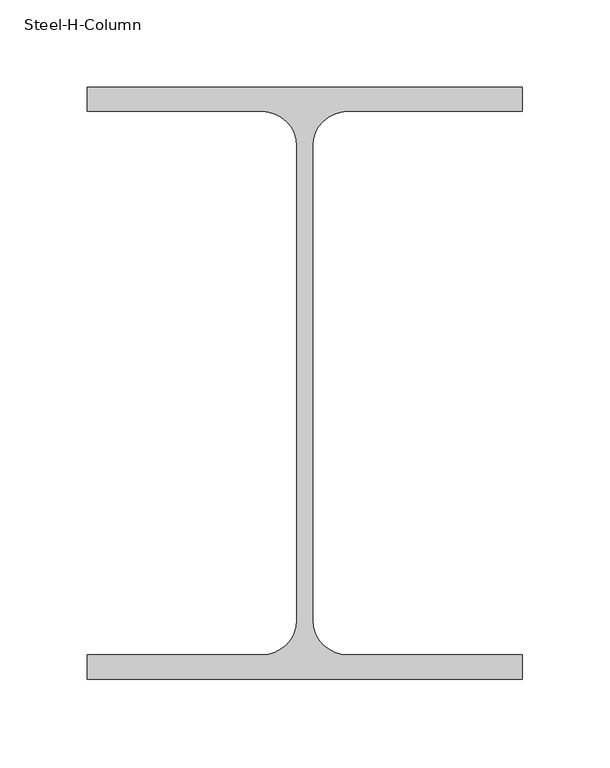
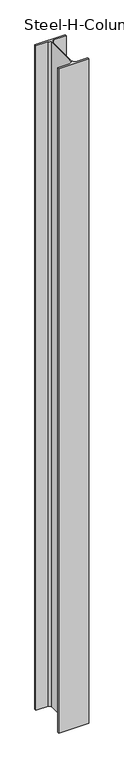
"""IFC4 building model written with IfcOpenShell, lengths in millimetres: column geometry, Steel-H-Column : CL121_H-340×250x9x14."""

import ifcopenshell
import ifcopenshell.guid

model = None  # the IFC model being written
_history = None  # IfcOwnerHistory: only IFC2X3 demands one
_inside = {}  # id of a spatial element -> (the spatial element, [elements in it])
_under = {}  # id of a project, library or spatial element -> (it, [spatial elements below it])
_declared = {}  # id of a project -> (the project, [libraries it declares])
_typed = {}  # id of a type object -> (the type object, [elements of that type])
_made_of = {}  # id of a material, layer set ... -> (it, [elements and type objects made of it])


def new_model(schema):
    """Start an empty IFC model of exactly this schema.

    Asked for "IFC4X3", IfcOpenShell would pick the latest addendum, in which some entities
    have other attributes; the version numbers below select the first issue.
    IFC2X3 requires an IfcOwnerHistory on every rooted entity: one is made here for all.
    """
    global model, _history
    if schema == "IFC4X3":
        model = ifcopenshell.file(schema_version=(4, 3, 0, 0))
    else:
        model = ifcopenshell.file(schema=schema)
    _inside.clear()
    _under.clear()
    _declared.clear()
    _typed.clear()
    _made_of.clear()
    _history = None
    if model.schema == "IFC2X3":
        org = make("IfcOrganization", Name="unknown")
        user = make(
            "IfcPersonAndOrganization",
            ThePerson=make("IfcPerson", FamilyName="unknown"),
            TheOrganization=org,
        )
        app = make(
            "IfcApplication",
            ApplicationDeveloper=org,
            Version="unknown",
            ApplicationFullName="unknown",
            ApplicationIdentifier="unknown",
        )
        _history = make(
            "IfcOwnerHistory",
            OwningUser=user,
            OwningApplication=app,
            ChangeAction="ADDED",
            CreationDate=0,
        )
    return model


def make(cls, **values):
    """One entity of the class cls with the attributes given. An attribute that is None is left unset."""
    return model.create_entity(
        cls, **{name: value for name, value in values.items() if value is not None}
    )


def rooted(cls, **values):
    """An entity with a GlobalId (a new one), such as an element, a storey or a relation."""
    return make(cls, GlobalId=ifcopenshell.guid.new(), OwnerHistory=_history, **values)


def si_unit(unit_type, name, prefix=None):
    """IfcSIUnit, for example si_unit("LENGTHUNIT", "METRE", prefix="MILLI")."""
    return make("IfcSIUnit", UnitType=unit_type, Prefix=prefix, Name=name)


def assignment(units):
    """IfcUnitAssignment: the units of a project."""
    return None if units is None else make("IfcUnitAssignment", Units=units)


def point(xyz):
    """IfcCartesianPoint."""
    return None if xyz is None else make("IfcCartesianPoint", Coordinates=xyz)


def direction(xyz):
    """IfcDirection."""
    return None if xyz is None else make("IfcDirection", DirectionRatios=xyz)


def frame(location, z_axis=None, x_axis=None):
    """IfcAxis2Placement3D, a coordinate frame: its origin and axes. An axis left out is left unset."""
    return make(
        "IfcAxis2Placement3D",
        Location=point(location),
        Axis=direction(z_axis),
        RefDirection=direction(x_axis),
    )


def frame_2d(location, x_axis=None):
    """IfcAxis2Placement2D, a coordinate frame in the plane: its origin and x axis."""
    return make(
        "IfcAxis2Placement2D", Location=point(location), RefDirection=direction(x_axis)
    )


def origin():
    """The frame at (0, 0, 0) with its axes left unset."""
    return frame((0.0, 0.0, 0.0))


def place(relative_to, where):
    """IfcLocalPlacement: puts the frame where relative to a parent placement (None: the world)."""
    return make(
        "IfcLocalPlacement", PlacementRelTo=relative_to, RelativePlacement=where
    )


def context(
    kind, dimensions, precision=None, world=None, true_north=None, identifier=None
):
    """IfcGeometricRepresentationContext, for example the 3D "Model" context."""
    return make(
        "IfcGeometricRepresentationContext",
        ContextIdentifier=identifier,
        ContextType=kind,
        CoordinateSpaceDimension=dimensions,
        Precision=precision,
        WorldCoordinateSystem=world,
        TrueNorth=true_north,
    )


def project(units=None, contexts=None):
    """IfcProject with its units and contexts."""
    return rooted(
        "IfcProject",
        Name="project",
        RepresentationContexts=contexts,
        UnitsInContext=assignment(units),
    )


def spatial(cls, under=None, at=None, **own):
    """A site, building, storey or space (cls), placed at a placement, below another one or the project."""
    s = rooted(cls, ObjectPlacement=at, **own)
    if under is not None:
        _under.setdefault(under.id(), (under, []))[1].append(s)
    return s


def polyline(points):
    """IfcPolyline through the points."""
    return make("IfcPolyline", Points=[point(p) for p in points])


def circle_curve(where, radius):
    """IfcCircle in the frame where."""
    return make("IfcCircle", Position=where, Radius=radius)


def trimmed(basis, trim1, trim2, sense, master):
    """IfcTrimmedCurve: the piece of a basis curve between two trims."""
    return make(
        "IfcTrimmedCurve",
        BasisCurve=basis,
        Trim1=trim1,
        Trim2=trim2,
        SenseAgreement=sense,
        MasterRepresentation=master,
    )


def segment(curve, same_sense, transition):
    """IfcCompositeCurveSegment."""
    return make(
        "IfcCompositeCurveSegment",
        Transition=transition,
        SameSense=same_sense,
        ParentCurve=curve,
    )


def composite_curve(segments, self_intersect=None):
    """IfcCompositeCurve: segments joined end to end."""
    return make("IfcCompositeCurve", Segments=segments, SelfIntersect=self_intersect)


def outline(outer, holes=None, kind="AREA"):
    """IfcArbitraryClosedProfileDef: a profile drawn as a closed curve; with holes, ...WithVoids."""
    if holes is None:
        return make("IfcArbitraryClosedProfileDef", ProfileType=kind, OuterCurve=outer)
    return make(
        "IfcArbitraryProfileDefWithVoids",
        ProfileType=kind,
        OuterCurve=outer,
        InnerCurves=holes,
    )


def extrude(swept, where, along, depth):
    """IfcExtrudedAreaSolid: the profile swept, set in the frame where, extruded along a direction by depth."""
    return make(
        "IfcExtrudedAreaSolid",
        SweptArea=swept,
        Position=where,
        ExtrudedDirection=direction(along),
        Depth=depth,
    )


def shape(context_of_items, identifier, shape_type, items):
    """IfcShapeRepresentation: the items that make up one representation, for example the "Body"."""
    return make(
        "IfcShapeRepresentation",
        ContextOfItems=context_of_items,
        RepresentationIdentifier=identifier,
        RepresentationType=shape_type,
        Items=items,
    )


def source(mapping_origin, context_of_items, identifier, shape_type, items):
    """IfcRepresentationMap: a shape defined once, which mapped items show again and again."""
    return make(
        "IfcRepresentationMap",
        MappingOrigin=mapping_origin,
        MappedRepresentation=shape(context_of_items, identifier, shape_type, items),
    )


def transform(
    local_origin,
    x_axis=None,
    y_axis=None,
    z_axis=None,
    scale=None,
    scale2=None,
    scale3=None,
    uniform=True,
):
    """IfcCartesianTransformationOperator3D, or its non-uniform kind. x_axis, y_axis, z_axis: its Axis1, 2, 3."""
    if uniform:
        return make(
            "IfcCartesianTransformationOperator3D",
            Axis1=direction(x_axis),
            Axis2=direction(y_axis),
            LocalOrigin=point(local_origin),
            Scale=scale,
            Axis3=direction(z_axis),
        )
    return make(
        "IfcCartesianTransformationOperator3DnonUniform",
        Axis1=direction(x_axis),
        Axis2=direction(y_axis),
        LocalOrigin=point(local_origin),
        Scale=scale,
        Axis3=direction(z_axis),
        Scale2=scale2,
        Scale3=scale3,
    )


def mapped(mapping_source, mapping_target):
    """IfcMappedItem: shows the shape of a source again, moved by a transform."""
    return make(
        "IfcMappedItem", MappingSource=mapping_source, MappingTarget=mapping_target
    )


def made_of(thing, what):
    """Note that an element or type object is made of a material, layer set ...; save() writes the relation."""
    if what is not None:
        _made_of.setdefault(what.id(), (what, []))[1].append(thing)
    return thing


def element(
    cls,
    number,
    at=None,
    inside=None,
    cuts=None,
    type_object=None,
    material=None,
    context=None,
    identifier="Body",
    shape_type=None,
    held_by="IfcProductDefinitionShape",
    body=None,
    shapes=None,
    **own,
):
    """One element of the class cls, such as IfcWall. Its Tag is "e" and its number.

    at: its placement. inside: the storey or other place that contains it. cuts: it is an
    opening in that element (IfcRelVoidsElement). A single representation is given by context,
    identifier, shape_type and body (its items); several are given by shapes. held_by: the class
    of the entity that holds the representations. save() writes the other relations.
    """
    e = rooted(cls, Tag="e%d" % number, ObjectPlacement=at, **own)
    if body is not None:
        shapes = [shape(context, identifier, shape_type, body)]
    if shapes is not None:
        e.Representation = make(held_by, Representations=shapes)
    if inside is not None:
        _inside.setdefault(inside.id(), (inside, []))[1].append(e)
    if cuts is not None:
        rooted(
            "IfcRelVoidsElement", RelatingBuildingElement=cuts, RelatedOpeningElement=e
        )
    if type_object is not None:
        _typed.setdefault(type_object.id(), (type_object, []))[1].append(e)
    return made_of(e, material)


def aggregate(whole, parts):
    """IfcRelAggregates: a whole, such as a stair, and the parts it consists of."""
    return rooted("IfcRelAggregates", RelatingObject=whole, RelatedObjects=parts)


def save(model, path):
    """Write the relations noted so far, then the file.

    IfcRelAggregates (storeys below a building ...), IfcRelContainedInSpatialStructure (elements
    in a storey), IfcRelDefinesByType, IfcRelAssociatesMaterial and IfcRelDeclares: one each for
    every whole, place, type object, material and project.
    """
    for whole, parts in _under.values():
        aggregate(whole, parts)
    for where, things in _inside.values():
        rooted(
            "IfcRelContainedInSpatialStructure",
            RelatedElements=things,
            RelatingStructure=where,
        )
    for kind, things in _typed.values():
        rooted("IfcRelDefinesByType", RelatedObjects=things, RelatingType=kind)
    for what, things in _made_of.values():
        rooted("IfcRelAssociatesMaterial", RelatedObjects=things, RelatingMaterial=what)
    for by, libraries in _declared.values():
        rooted("IfcRelDeclares", RelatingContext=by, RelatedDefinitions=libraries)
    model.write(path)


def steel_h_column_09ca9198(model_context):
    return source(origin(), model_context, "Body", "SweptSolid", [
        extrude(outline(composite_curve([segment(polyline([(125.0, 170.0), (125.0, 156.0), (24.5, 156.0)]), True, "CONTINUOUS"), segment(trimmed(circle_curve(frame_2d((24.5, 136.0)), 20.0), [point((24.5, 156.0))], [point((4.5, 136.0))], True, "CARTESIAN"), True, "CONTINUOUS"), segment(polyline([(4.5, 136.0), (4.5, -136.0)]), True, "CONTINUOUS"), segment(trimmed(circle_curve(frame_2d((24.5, -136.0)), 20.0), [point((4.5, -136.0))], [point((24.5, -156.0))], True, "CARTESIAN"), True, "CONTINUOUS"), segment(polyline([(24.5, -156.0), (125.0, -156.0), (125.0, -170.0), (-125.0, -170.0), (-125.0, -156.0), (-24.5, -156.0)]), True, "CONTINUOUS"), segment(trimmed(circle_curve(frame_2d((-24.5, -136.0)), 20.0), [point((-24.5, -156.0))], [point((-4.5, -136.0))], True, "CARTESIAN"), True, "CONTINUOUS"), segment(polyline([(-4.5, -136.0), (-4.5, 136.0)]), True, "CONTINUOUS"), segment(trimmed(circle_curve(frame_2d((-24.5, 136.0)), 20.0), [point((-4.5, 136.0))], [point((-24.5, 156.0))], True, "CARTESIAN"), True, "CONTINUOUS"), segment(polyline([(-24.5, 156.0), (-125.0, 156.0), (-125.0, 170.0), (125.0, 170.0)]), True, "CONTINUOUS")], self_intersect=False)), frame((0.0, 0.0, 200.0), z_axis=(0.0, 0.0, 1.0), x_axis=(1.0, 0.0, 0.0)), (0.0, 0.0, 1.0), 5800.0),
    ])


if __name__ == "__main__":
    model = new_model("IFC4")
    model_context = context("Model", 3, world=origin())
    ifc_project = project(units=[si_unit("LENGTHUNIT", "METRE", prefix="MILLI")], contexts=[model_context])
    site = spatial("IfcSite", under=ifc_project)
    building = spatial("IfcBuilding", under=site)
    placement = place(None, origin())
    steel_h_column_shape = steel_h_column_09ca9198(model_context)
    element("IfcColumn", 1, ObjectType="Steel-H-Column : CL121_H-340×250x9x14", at=placement, inside=building, context=model_context, shape_type="MappedRepresentation", body=[
        mapped(steel_h_column_shape, transform((0.0, 0.0, 0.0), x_axis=(1.0, 0.0, 0.0), y_axis=(0.0, 1.0, 0.0), z_axis=(0.0, 0.0, 1.0))),
    ])
    save(model, "model.ifc")

# Revit data of these elements
# Project information
#   Project ISM Data = "<?xml version=\"1.0\" encoding=\"utf-16\"?><ism schema_version=\"03.00\"><section_positioning><element family_name=\"CO_RC_REC\" symbol_name=\"CCC12_Rec_450x450\" section_id=\"F2ADF140-E21A-4820-8170-6F63D956DCAD\" category=\"OST_StructuralColumns\" mirror_y=\"0\" mirror_x=\"0\" /><element family_name=\"CO_RC_REC\" symbol_name=\"CCC12_Rec_450x450\" section_id=\"B35A310E-4F33-462b-819C-3ADD300C0CEB\" category=\"OST_StructuralColumns\" mirror_y=\"0\" mirror_x=\"0\" /><element family_name=\"CO_RC_REC\" symbol_name=\"CCC12_Rec_450x450\" section_id=\"711054EC-0DB2-46e3-AD20-004560300C00\" category=\"OST_StructuralColumns\" mirror_y=\"0\" mirror_x=\"0\" /><element family_name=\"CO_RC_REC\" symbol_name=\"300 x 450\" section_id=\"B5C54EC9-8EBD-4860-AB72-EF5791AED394\" category=\"OST_StructuralColumns\" mirror_y=\"0\" mirror_x=\"0\" /><element family_name=\"GI_RC_C\" symbol_name=\"SGC11_400x500\" section_id=\"0A7B8D02-9EA4-4aa9-A41A-E30BB5B6B6C5\" category=\"OST_StructuralFraming\" mirror_y=\"0\" mirror_x=\"0\" /><element family_name=\"GI_RC_C\" symbol_name=\"SGC11_400x500\" section_id=\"714BBD27-DB58-47da-B54C-5806291C2D3C\" category=\"OST_StructuralFraming\" mirror_y=\"0\" mirror_x=\"0\" /><element family_name=\"GI_RC_C\" symbol_name=\"SGC11_400x500\" section_id=\"F36E62C1-13EE-4807-A3C1-899E23E0BEDE\" category=\"OST_StructuralFraming\" mirror_y=\"0\" mirror_x=\"0\" /><element family_name=\"GI_RC_C\" symbol_name=\"SGC11_400x500\" section_id=\"F5448801-679E-44d6-8F46-E676344F8165\" category=\"OST_StructuralFraming\" mirror_y=\"0\" mirror_x=\"0\" /><element family_name=\"GI_RC_C\" symbol_name=\"SGC11_400x600\" section_id=\"05D74241-6318-4cac-95F5-7B878260D5B5\" category=\"OST_StructuralFraming\" mirror_y=\"0\" mirror_x=\"0\" /><element family_name=\"GI_RC_C\" symbol_name=\"SGC11_400x500\" section_id=\"846DCB0C-E06B-4978-9D43-E1CC0FDE7595\" category=\"OST_StructuralFraming\" mirror_y=\"0\" mirror_x=\"0\" /><element family_name=\"GI_RC_C\" symbol_name=\"SGC11_400x500\" section_id=\"2ADF82B8-986D-4f44-85DE-89D921292160\" category=\"OST_StructuralFraming\" mirror_y=\"0\" mirror_x=\"0\" /><element family_name=\"GI_RC_C\" symbol_name=\"SGC11_400x500\" section_id=\"7AF371ED-051B-4a30-8826-11F11C212B73\" category=\"OST_StructuralFraming\" mirror_y=\"0\" mirror_x=\"0\" /><element family_name=\"GI_RC_C\" symbol_name=\"SGC11_400x500\" section_id=\"2FE74006-ADDA-412f-A522-853919E62B4D\" category=\"OST_StructuralFraming\" mirror_y=\"0\" mirror_x=\"0\" /><element family_name=\"GI_RC_C\" symbol_name=\"SGC11_400x500\" section_id=\"09B63641-D581-4a6c-A18E-54C17EC989A4\" category=\"OST_StructuralFraming\" mirror_y=\"0\" mirror_x=\"0\" /><element family_name=\"GI_RC_C\" symbol_name=\"SGC11_400x500\" section_id=\"0DD6B52A-77D0-45a1-82B1-8236ED57078C\" category=\"OST_StructuralFraming\" mirror_y=\"0\" mirror_x=\"0\" /><element family_name=\"GI_RC_C\" symbol_name=\"SGC11_400x500\" section_id=\"35D311D2-DEB8-4469-97DE-110B6DF5B84D\" category=\"OST_StructuralFraming\" mirror_y=\"0\" mirror_x=\"0\" /><element family_name=\"GI_RC_C\" symbol_name=\"SGC11_400x500\" section_id=\"0D3CCDE5-CFF9-431b-A4BD-01BF6636D6BD\" category=\"OST_StructuralFraming\" mirror_y=\"0\" mirror_x=\"0\" /><element family_name=\"GI_RC_C\" symbol_name=\"SGC11_400x500\" section_id=\"C62B2A5B-024A-47ac-B030-C17A67E64A7B\" category=\"OST_StructuralFraming\" mirror_y=\"0\" mirror_x=\"0\" /><element family_name=\"GI_RC_C\" symbol_name=\"SGC11_400x500\" section_id=\"944C6E43-E607-48c3-8358-9E6CB88346E7\" category=\"OST_StructuralFraming\" mirror_y=\"0\" mirror_x=\"0\" /><element family_name=\"GI_RC_C\" symbol_name=\"SGC11_400x500\" section_id=\"A4B1F42D-B1C2-4ad2-8AD6-DB0D5E05998D\" category=\"OST_StructuralFraming\" mirror_y=\"0\" mirror_x=\"0\" /><element family_name=\"GI_RC_C\" symbol_name=\"SGC11_400x500\" section_id=\"007E6C70-1139-4b48-B003-C76FAD4C249A\" category=\"OST_StructuralFraming\" mirror_y=\"0\" mirror_x=\"0\" /><element family_name=\"GI_RC_C\" symbol_name=\"SGC11_400x500\" section_id=\"9941AC94-F03A-464c-9912-04590E0C31E0\" category=\"OST_StructuralFraming\" mirror_y=\"0\" mirror_x=\"0\" /><element family_name=\"GI_RC_C\" symbol_name=\"SGC11_400x500\" section_id=\"CFD98B8D-8FF4-4e71-A909-0FE7DBCE924E\" category=\"OST_StructuralFraming\" mirror_y=\"0\" mirror_x=\"0\" /><element family_name=\"GI_RC_C\" symbol_name=\"SGC11_400x500\" section_id=\"58262161-98E6-45c8-B2BD-4508105FF662\" category=\"OST_StructuralFraming\" mirror_y=\"0\" mirror_x=\"0\" /><element family_name=\"GI_RC_C\" symbol_name=\"SGC11_400x500\" section_id=\"66AB4841-610A-4883-97F7-1282A56484E1\" category=\"OST_StructuralFraming\" mirror_y=\"0\" mirror_x=\"0\" /><element family_name=\"GI_RC_C\" symbol_name=\"SGC11_400x500\" section_id=\"D2B324BE-BBD6-49da-9730-60EA7AD4D3A0\" category=\"OST_StructuralFraming\" mirror_y=\"0\" mirror_x=\"0\" /><element family_name=\"GI_RC_C\" symbol_name=\"SGC11_400x500\" section_id=\"92A8ECE7-C053-46b1-92ED-F2C041617E7B\" category=\"OST_StructuralFraming\" mirror_y=\"0\" mirror_x=\"0\" /><element family_name=\"GI_RC_C\" symbol_name=\"SGC11_400x500\" section_id=\"B4C4BDB0-65C4-4016-9C78-DBD77E229523\" category=\"OST_StructuralFraming\" mirror_y=\"0\" mirror_x=\"0\" /><element family_name=\"GI_RC_C\" symbol_name=\"SGC11_400x500\" section_id=\"57270646-162F-4c83-BDB7-A5FBEA9120BD\" category=\"OST_StructuralFraming\" mirror_y=\"0\" mirror_x=\"0\" /><element family_name=\"GI_RC_C\" symbol_name=\"SGC11_400x500\" section_id=\"BDEF733F-00AA-4eee-B6C6-50229FC1D236\" category=\"OST_StructuralFraming\" mirror_y=\"0\" mirror_x=\"0\" /><element family_name=\"GI_RC_C\" symbol_name=\"SGC11_400x500\" section_id=\"84A94E1E-3074-40f4-9690-97191755F019\" category=\"OST_StructuralFraming\" mirror_y=\"0\" mirror_x=\"0\" /><element family_name=\"GI_RC_C\" symbol_name=\"SGC11_400x500\" section_id=\"8A7D913D-7967-4718-912D-B83DF0AD2EDD\" category=\"OST_StructuralFraming\" mirror_y=\"0\" mirror_x=\"0\" /><element family_name=\"GI_RC_C\" symbol_name=\"SGC11_400x500\" section_id=\"83553D70-90FA-469c-B5C3-EF03F3FC6475\" category=\"OST_StructuralFraming\" mirror_y=\"0\" mirror_x=\"0\" /><element family_name=\"GI_RC_C\" symbol_name=\"SGC11_400x500\" section_id=\"6880C1E4-C50B-4c1b-B61C-23F2D8C46873\" category=\"OST_StructuralFraming\" mirror_y=\"0\" mirror_x=\"0\" /><element family_name=\"GI_RC_C\" symbol_name=\"SGC11_400x500\" section_id=\"08594C43-CD40-47de-A3BA-8BFB47F64994\" category=\"OST_StructuralFraming\" mirror_y=\"0\" mirror_x=\"0\" /><element family_name=\"GI_RC_C\" symbol_name=\"SGC11_400x500\" section_id=\"7D2E11FA-A5E1-4434-B9BE-AABA1A16CA03\" category=\"OST_StructuralFraming\" mirror_y=\"0\" mirror_x=\"0\" /><element family_name=\"GI_RC_C\" symbol_name=\"SGC11_400x500\" section_id=\"D892DFA4-5441-4ad2-A390-253492293B1B\" category=\"OST_StructuralFraming\" mirror_y=\"0\" mirror_x=\"0\" /><element family_name=\"GI_RC_C\" symbol_name=\"SGC11_400x500\" section_id=\"E5A32FE6-89C4-49f1-B3B9-1CABE7C48A4D\" category=\"OST_StructuralFraming\" mirror_y=\"0\" mirror_x=\"0\" /><element family_name=\"GI_RC_C\" symbol_name=\"SGC11_400x500\" section_id=\"8AE872C2-5DBE-47c5-934B-7E964A84B589\" category=\"OST_StructuralFraming\" mirror_y=\"0\" mirror_x=\"0\" /><element family_name=\"GI_RC_C\" symbol_name=\"SGC11_400x500\" section_id=\"3C847B60-488A-4604-A400-16A3A65E919B\" category=\"OST_StructuralFraming\" mirror_y=\"0\" mirror_x=\"0\" /><element family_name=\"GI_RC_C\" symbol_name=\"SGC11_400x500\" section_id=\"DBEC432A-3F7B-4266-AD99-2A937DC70BCF\" category=\"OST_StructuralFraming\" mirror_y=\"0\" mirror_x=\"0\" /><element family_name=\"GI_RC_C\" symbol_name=\"SGC11_400x500\" section_id=\"59403DD6-7A51-48aa-A3BE-962457E6F10E\" category=\"OST_StructuralFraming\" mirror_y=\"0\" mirror_x=\"0\" /><element family_name=\"GI_RC_C\" symbol_name=\"SGC11_400x500\" section_id=\"11CDDF5D-38B6-43b2-A291-FC188BE232BC\" category=\"OST_StructuralFraming\" mirror_y=\"0\" mirror_x=\"0\" /><element family_name=\"GI_RC_C\" symbol_name=\"SGC11_400x500\" section_id=\"10BF2843-EFC9-4136-933C-5B270D970277\" category=\"OST_StructuralFraming\" mirror_y=\"0\" mirror_x=\"0\" /><element family_name=\"GI_RC_C\" symbol_name=\"SGC11_400x500\" section_id=\"E1B09A9C-F6C6-47d9-976B-E313C0E3F52B\" category=\"OST_StructuralFraming\" mirror_y=\"0\" mirror_x=\"0\" /><element family_name=\"GI_RC_C\" symbol_name=\"SGC11_400x500\" section_id=\"A3A22EC3-26C8-4588-A0AB-AFAE02DF267E\" category=\"OST_StructuralFraming\" mirror_y=\"0\" mirror_x=\"0\" /><element family_name=\"GI_RC_C\" symbol_name=\"SGC11_400x500\" section_id=\"114828FC-BDC1-4343-9119-BCB5395DAA64\" category=\"OST_StructuralFraming\" mirror_y=\"0\" mirror_x=\"0\" /><element family_name=\"GI_RC_C\" symbol_name=\"SGC11_400x500\" section_id=\"797626F9-3558-4623-826F-15FB93088CB3\" category=\"OST_StructuralFraming\" mirror_y=\"0\" mirror_x=\"0\" /><element family_name=\"GI_RC_C\" symbol_name=\"SGC11_400x500\" section_id=\"4BF369CD-DF09-4346-96CB-C6C6380A2599\" category=\"OST_StructuralFraming\" mirror_y=\"0\" mirror_x=\"0\" /><element family_name=\"GI_RC_C\" symbol_name=\"SGC11_400x500\" section_id=\"722B46BA-61C4-44a1-9ECF-325B60B6688D\" category=\"OST_StructuralFraming\" mirror_y=\"0\" mirror_x=\"0\" /><element family_name=\"GI_RC_C\" symbol_name=\"SGC11_400x500\" section_id=\"C33DBE84-19C1-4379-AB6E-A41F7420F18C\" category=\"OST_StructuralFraming\" mirror_y=\"0\" mirror_x=\"0\" /><element family_name=\"GI_RC_C\" symbol_name=\"SGC11_400x500\" section_id=\"1F2D3B75-66F2-4d88-A1DD-647969477B86\" category=\"OST_StructuralFraming\" mirror_y=\"0\" mirror_x=\"0\" /><element family_name=\"GI_RC_C\" symbol_name=\"SGC11_400x500\" section_id=\"DFBF96B2-410A-4f39-80C4-D8CF78561C93\" category=\"OST_StructuralFraming\" mirror_y=\"0\" mirror_x=\"0\" /><element family_name=\"GI_RC_C\" symbol_name=\"SGC11_400x500\" section_id=\"D6793CD3-AB64-417c-9C28-8B18A0A2D336\" category=\"OST_StructuralFraming\" mirror_y=\"0\" mirror_x=\"0\" /><element family_name=\"GI_RC_C\" symbol_name=\"SGC11_400x500\" section_id=\"90884AC0-EA00-4caa-86E1-E6B886FD90ED\" category=\"OST_StructuralFraming\" mirror_y=\"0\" mirror_x=\"0\" /><element family_name=\"GI_RC_C\" symbol_name=\"SGC11_400x500\" section_id=\"64BC7B89-F7C8-4dae-A5C8-F10DF9E5F6BA\" category=\"OST_StructuralFraming\" mirror_y=\"0\" mirror_x=\"0\" /><element family_name=\"GI_RC_C\" symbol_name=\"SGC11_400x500\" section_id=\"D82E4D85-2728-40e5-9F60-1C7FB2990D78\" category=\"OST_StructuralFraming\" mirror_y=\"0\" mirror_x=\"0\" /><element family_name=\"GI_RC_C\" symbol_name=\"SGC11_400x500\" section_id=\"1E6D05B9-BF84-4669-AA27-948ADA1D511E\" category=\"OST_StructuralFraming\" mirror_y=\"0\" mirror_x=\"0\" /><element family_name=\"GI_RC_C\" symbol_name=\"SGC11_400x500\" section_id=\"73608CB2-EB94-466e-883D-814030EF49D6\" category=\"OST_StructuralFraming\" mirror_y=\"0\" mirror_x=\"0\" /><element family_name=\"GI_RC_C\" symbol_name=\"SGC11_400x500\" section_id=\"4EAF07EF-4E08-4065-9F08-BF69D4413867\" category=\"OST_StructuralFraming\" mirror_y=\"1\" mirror_x=\"1\" /></section_positioning><surface_member_mappings /><element_binding><element revit_id=\"0aa8b22b-49cd-4eb2-b994-d423f7aad482-0014435e\" ism_id=\"637A3C89-B4B9-4EE4-9E04-FF73E7A5771D\" /><element revit_id=\"af7cfdda-f71a-4a09-bb03-63e0c16d5d93-00152efa\" ism_id=\"088C1743-AFAE-4D55-B14F-2330F3A79060\" /><element revit_id=\"af7cfdda-f71a-4a09-bb03-63e0c16d5d93-00152efc\" ism_id=\"38278b30-864a-4bde-bfee-6c2d4309b281\" /><element revit_id=\"af7cfdda-f71a-4a09-bb03-63e0c16d5d93-00152eff\" ism_id=\"e2895b00-887b-4cf1-92a9-c4855f67b579\" /><element revit_id=\"af7cfdda-f71a-4a09-bb03-63e0c16d5d93-00152f02\" ism_id=\"a6b13b86-1938-47ee-8937-754844bb71d9\" /><element revit_id=\"af7cfdda-f71a-4a09-bb03-63e0c16d5d93-00152f05\" ism_id=\"b3cdb4ae-01be-49a8-8521-dfb37fcb7a09\" /><element revit_id=\"af7cfdda-f71a-4a09-bb03-63e0c16d5d93-00152f08\" ism_id=\"0a200294-2d0f-43b2-a10b-c345be42008c\" /><element revit_id=\"af7cfdda-f71a-4a09-bb03-63e0c16d5d
#     93-00152f0a\" ism_id=\"434ac00d-0b75-408a-b526-bf8655b26baf\" /><element revit_id=\"af7cfdda-f71a-4a09-bb03-63e0c16d5d93-00152f0c\" ism_id=\"5e4f7e2a-2154-47cc-93bc-24e7bd197632\" /><element revit_id=\"af7cfdda-f71a-4a09-bb03-63e0c16d5d93-00152f0e\" ism_id=\"f1998cd9-044c-4f7a-99e6-248bc5b45dba\" /><element revit_id=\"af7cfdda-f71a-4a09-bb03-63e0c16d5d93-00152f10\" ism_id=\"6ca0e144-6dd7-4824-b6a4-c3599ffcc64c\" /><element revit_id=\"af7cfdda-f71a-4a09-bb03-63e0c16d5d93-00152f12\" ism_id=\"173f1f07-ca52-4750-b7f6-1ef0180c36ba\" /><element revit_id=\"af7cfdda-f71a-4a09-bb03-63e0c16d5d93-00152f15\" ism_id=\"29a619d1-86ac-46c7-a220-2e78769b313e\" /><element revit_id=\"af7cfdda-f71a-4a09-bb03-63e0c16d5d93-00152f17\" ism_id=\"de21b25d-6b5e-4da6-89ee-8b671f1287ec\" /><element revit_id=\"af7cfdda-f71a-4a09-bb03-63e0c16d5d93-00152f19\" ism_id=\"70cdf538-eeaa-48c4-9315-181e56578638\" /><element revit_id=\"af7cfdda-f71a-4a09-bb03-63e0c16d5d93-00152f1b\" ism_id=\"49734cf8-a963-4163-b104-a25bff74fff0\" /><element revit_id=\"af7cfdda-f71a-4a09-bb03-63e0c16d5d93-00152f1d\" ism_id=\"a5a98e28-e98d-4759-bcab-d40632bfc19f\" /><element revit_id=\"af7cfdda-f71a-4a09-bb03-63e0c16d5d93-00152f1f\" ism_id=\"ab6af08f-90da-4d2f-a66a-db65621b8e94\" /><element revit_id=\"af7cfdda-f71a-4a09-bb03-63e0c16d5d93-00152f21\" ism_id=\"a65b64ab-134d-4223-82b7-5e66d90bc276\" /><element revit_id=\"af7cfdda-f71a-4a09-bb03-63e0c16d5d93-00152f23\" ism_id=\"6a1f317f-8940-4af8-9522-8e6c47c0c3a6\" /><element revit_id=\"af7cfdda-f71a-4a09-bb03-63e0c16d5d93-00152f25\" ism_id=\"880c6aab-7058-4382-9d83-6c759bdcf822\" /><element revit_id=\"af7cfdda-f71a-4a09-bb03-63e0c16d5d93-00152f27\" ism_id=\"555977b1-6494-4ee8-b235-8bae97762787\" /><element revit_id=\"af7cfdda-f71a-4a09-bb03-63e0c16d5d93-00152f29\" ism_id=\"66c9b467-8c65-4f1e-9542-95b43d793e9b\" /><element revit_id=\"af7cfdda-f71a-4a09-bb03-63e0c16d5d93-00152f2b\" ism_id=\"217a9ce2-64ab-4115-836e-06014fa1b21e\" /><element revit_id=\"af7cfdda-f71a-4a09-bb03-63e0c16d5d93-00152f2d\" ism_id=\"f7fc30da-832d-44e7-bab3-dd115d25639e\" /><element revit_id=\"af7cfdda-f71a-4a09-bb03-63e0c16d5d93-00152f2f\" ism_id=\"715eb46c-1b8d-4226-a7c6-6c6c165bf34d\" /><element revit_id=\"af7cfdda-f71a-4a09-bb03-63e0c16d5d93-00152f31\" ism_id=\"ef53c2b2-6fcf-42d2-96ea-f30a899bf64f\" /><element revit_id=\"af7cfdda-f71a-4a09-bb03-63e0c16d5d93-00152f34\" ism_id=\"1aefa093-18ee-4a97-8178-1b1fb4b7aceb\" /><element revit_id=\"af7cfdda-f71a-4a09-bb03-63e0c16d5d93-00152f38\" ism_id=\"262f02a9-64ca-487b-befd-4b58d44dffa7\" /><element revit_id=\"af7cfdda-f71a-4a09-bb03-63e0c16d5d93-00152f3b\" ism_id=\"6f2442a8-c4c0-4b53-9d7f-7059d6ededd2\" /><element revit_id=\"af7cfdda-f71a-4a09-bb03-63e0c16d5d93-00152f3e\" ism_id=\"dd838df4-69c7-406c-93e1-418c01f5734f\" /><element revit_id=\"af7cfdda-f71a-4a09-bb03-63e0c16d5d93-00152f40\" ism_id=\"9dec5077-28a7-4c32-95d2-08813de6a916\" /><element revit_id=\"af7cfdda-f71a-4a09-bb03-63e0c16d5d93-00152f42\" ism_id=\"9370ae5f-9277-4bb3-917b-cb3f318800a8\" /><element revit_id=\"af7cfdda-f71a-4a09-bb03-63e0c16d5d93-00152f44\" ism_id=\"0f3f2c81-58b4-4698-b1be-75061a4a2ae1\" /><element revit_id=\"af7cfdda-f71a-4a09-bb03-63e0c16d5d93-00152f46\" ism_id=\"95dca10f-6510-4ae7-a23e-7a1fd6939662\" /><element revit_id=\"af7cfdda-f71a-4a09-bb03-63e0c16d5d93-00152f49\" ism_id=\"83bad907-6a1c-4702-9990-a1a9c13d0160\" /><element revit_id=\"af7cfdda-f71a-4a09-bb03-63e0c16d5d93-00152f4d\" ism_id=\"7dba72dc-0de8-457c-8d3c-9c80941133ff\" /><element revit_id=\"af7cfdda-f71a-4a09-bb03-63e0c16d5d93-00152f51\" ism_id=\"a6cf3de2-949b-45b4-8029-061e06e5ab91\" /><element revit_id=\"af7cfdda-f71a-4a09-bb03-63e0c16d5d93-00152f54\" ism_id=\"77af5754-dd62-4c90-accb-d0b9405b5baf\" /><element revit_id=\"af7cfdda-f71a-4a09-bb03-63e0c16d5d93-00152f56\" ism_id=\"6461cb37-823d-49bb-bea2-3dbd4db85a81\" /><element revit_id=\"af7cfdda-f71a-4a09-bb03-63e0c16d5d93-00152f59\" ism_id=\"e2f2909f-27bc-426e-b2db-27b1217d3560\" /><element revit_id=\"af7cfdda-f71a-4a09-bb03-63e0c16d5d93-00152f5b\" ism_id=\"46c410de-fc65-4593-ae24-da1a154b45fb\" /><element revit_id=\"af7cfdda-f71a-4a09-bb03-63e0c16d5d93-00152f5d\" ism_id=\"d7d73cf7-a31f-421c-bc39-3ba338a334b1\" /><element revit_id=\"af7cfdda-f71a-4a09-bb03-63e0c16d5d93-00152f61\" ism_id=\"6bd81f7b-5fd8-4f19-ad3a-4e009274854c\" /><element revit_id=\"af7cfdda-f71a-4a09-bb03-63e0c16d5d93-00152f64\" ism_id=\"f25b9af0-504f-4aaf-a359-d2bc9d32b683\" /><element revit_id=\"af7cfdda-f71a-4a09-bb03-63e0c16d5d93-00152f66\" ism_id=\"f143dcd3-1cc7-47ae-b4ed-c960a7d1349c\" /><element revit_id=\"af7cfdda-f71a-4a09-bb03-63e0c16d5d93-00152f68\" ism_id=\"296e8d7f-a89b-405a-b793-fc1ea4b11be5\" /><element revit_id=\"af7cfdda-f71a-4a09-bb03-63e0c16d5d93-00152f6b\" ism_id=\"48b24488-3184-439c-b285-73e81edfef17\" /><element revit_id=\"af7cfdda-f71a-4a09-bb03-63e0c16d5d93-00152f6e\" ism_id=\"0db0ccd4-631c-4972-aad8-2fd483c55629\" /><element revit_id=\"af7cfdda-f71a-4a09-bb03-63e0c16d5d93-00152f71\" ism_id=\"ee51bd40-01d8-4a48-92c6-90509a96cad2\" /><element revit_id=\"af7cfdda-f71a-4a09-bb03-63e0c16d5d93-00152f73\" ism_id=\"e5c66ce6-ca9d-4591-9d75-5348307a88bc\" /><element revit_id=\"af7cfdda-f71a-4a09-bb03-63e0c16d5d93-00152f75\" ism_id=\"892d82ae-6f73-4af5-8575-78955f2b6c3b\" /><element revit_id=\"af7cfdda-f71a-4a09-bb03-63e0c16d5d93-00152f78\" ism_id=\"cb5b2a2e-5551-4b87-9d0b-6382c09e6ce2\" /><element revit_id=\"af7cfdda-f71a-4a09-bb03-63e0c16d5d93-00152f7c\" ism_id=\"1177c4ab-d04b-426b-80ba-afa1f1403e20\" /><element revit_id=\"af7cfdda-f71a-4a09-bb03-63e0c16d5d93-00152f7f\" ism_id=\"235d8a18-f10a-44ad-8945-ebb2f02646fa\" /><element revit_id=\"af7cfdda-f71a-4a09-bb03-63e0c16d5d93-00152f83\" ism_id=\"6127db9d-7d4b-44c8-806c-e4f7d278db0c\" /><element revit_id=\"af7cfdda-f71a-4a09-bb03-63e0c16d5d93-00152f86\" ism_id=\"85d79da8-d317-4e5b-88a2-88d20cb73d7d\" /><element revit_id=\"af7cfdda-f71a-4a09-bb03-63e0c16d5d93-00152f89\" ism_id=\"f4105a19-7c5e-4970-9446-50e578b67af2\" /><element revit_id=\"af7cfdda-f71a-4a09-bb03-63e0c16d5d93-00152f8b\" ism_id=\"ab299061-87b1-4edc-8a5c-c55542368f39\" /><element revit_id=\"af7cfdda-f71a-4a09-bb03-63e0c16d5d93-00152f8d\" ism_id=\"43097401-25be-48d4-a7ba-f3c37c1b84e9\" /><element revit_id=\"af7cfdda-f71a-4a09-bb03-63e0c16d5d93-00152f8f\" ism_id=\"fd9214b7-59e9-4736-b544-a37d4c180e24\" /><element revit_id=\"af7cfdda-f71a-4a09-bb03-63e0c16d5d93-00152f91\" ism_id=\"b83d1d95-2d97-4532-8a94-368577601c17\" /><element revit_id=\"af7cfdda-f71a-4a09-bb03-63e0c16d5d93-00152f94\" ism_id=\"9bd5e620-e2eb-4ede-9a8b-b0183e171248\" /><element revit_id=\"af7cfdda-f71a-4a09-bb03-63e0c16d5d93-00152f97\" ism_id=\"d6f9d903-1605-43dc-872c-2f9de6642af6\" /><element revit_id=\"af7cfdda-f71a-4a09-bb03-63e0c16d5d93-00152f99\" ism_id=\"7c236b12-3da8-4ae0-bc99-2aa089118476\" /><element revit_id=\"af7cfdda-f71a-4a09-bb03-63e0c16d5d93-00152f9b\" ism_id=\"2b88d03d-aeef-4f51-b98c-562513d6f6da\" /><element revit_id=\"af7cfdda-f71a-4a09-bb03-63e0c16d5d93-00152f9d\" ism_id=\"6639b07f-6759-4580-bc0a-91cdbc82216d\" /><element revit_id=\"af7cfdda-f71a-4a09-bb03-63e0c16d5d93-00152f9f\" ism_id=\"d17e7cf5-d760-4c38-8bb0-8a57fe45e3ad\" /><element revit_id=\"af7cfdda-f71a-4a09-bb03-63e0c16d5d93-00152fa2\" ism_id=\"6dbdf2a2-22ac-4132-a9ae-8992fe15b0d7\" /><element revit_id=\"af7cfdda-f71a-4a09-bb03-63e0c16d5d93-00152fa4\" ism_id=\"663381be-9f3f-499f-b7c1-64170401ecb3\" /><element revit_id=\"af7cfdda-f71a-4a09-bb03-63e0c16d5d93-00152fa6\" ism_id=\"5ba3ff14-3d24-47a8-9418-aecce16bd943\" /><element revit_id=\"af7cfdda-f71a-4a09-bb03-63e0c16d5d93-00152fa8\" ism_id=\"8f845e6a-1432-4c61-8362-e12c105320fb\" /><element revit_id=\"af7cfdda-f71a-4a09-bb03-63e0c16d5d93-00152faa\" ism_id=\"263897bf-02c2-4ed7-8e3f-2020d545125e\" /><element revit_id=\"af7cfdda-f71a-4a09-bb03-63e0c16d5d93-00152fac\" ism_id=\"f1241312-d990-4c87-92ff-afc1975a3d67\" /><element revit_id=\"af7cfdda-f71a-4a09-bb03-63e0c16d5d93-00152fae\" ism_id=\"5740cb23-0cbc-47ce-acea-31b5a043bf0c\" /><element revit_id=\"af7cfdda-f71a-4a09-bb03-63e0c16d5d93-00152fb0\" ism_id=\"7aeaeafb-f9bc-4bee-b237-caade22069b8\" /><element revit_id=\"af7cfdda-f71a-4a09-bb03-63e0c16d5d93-00152fb3\" ism_id=\"90084dda-e197-4e46-8e5b-4f629a594830\" /><element revit_id=\"af7cfdda-f71a-4a09-bb03-63e0c16d5d93-00152fb5\" ism_id=\"2c392f12-2b50-4bd2-8c41-ef64640e587b\" /><element revit_id=\"af7cfdda-f71a-4a09-bb03-63e0c16d5d93-00152fb7\" ism_id=\"d25284c0-6931-4cbb-8ed3-63397f6a5616\" /><element revit_id=\"af7cfdda-f71a-4a09-bb03-63e0c16d5d93-00152fb9\" ism_id=\"32799d39-e9bc-468c-ac64-a3f2c8e075af\" /><element revit_id=\"af7cfdda-f71a-4a09-bb03-63e0c16d5d93-00152fbb\" ism_id=\"61a092b8-d924-4e61-a1ef-adc051541aaf\" /><element revit_id=\"af7cfdda-f71a-4a09-bb03-63e0c16d5d93-00152fbe\" ism_id=\"ae89ad42-0006-42ee-9328-01a896002b7a\" /><element revit_id=\"af7cfdda-f71a-4a09-bb03-63e0c16d5d93-00152fc0\" ism_id=\"7b4d47fd-5fcd-4692-9b39-36bb95372647\" /><element revit_id=\"af7cfdda-f71a-4a09-bb03-63e0c16d5d93-00152fc2\" ism_id=\"150f022d-eb78-47d8-8d70-c7ea5433f366\" /><element revit_id=\"af7cfdda-f71a-4a09-bb03-63e0c16d5d93-00152fc4\" ism_id=\"6780451e-52c6-4962-8bb4-f1fd57bf7865\" /><element revit_id=\"af7cfdda-f71a-4a09-bb03-63e0c16d5d93-00152fc6\" ism_id=\"b3896748-2d7c-424b-ae81-8b769d840fbc\" /><element revit_id=\"af7cfdda-f71a-4a09-bb03-63e0c16d5d93-00152fc9\" ism_id=\"0c64c745-ce95-4f37-8a9d-d07fd5d17ecb\" /><element revit_id=\"af7cfdda-f71a-4a09-bb03-63e0c16d5d93-00152fcc\" ism_id=\"dc23390d-d501-4d7e-9369-f7793a7306a7\" /><element revit_id=\"af7cfdda-f71a-4a09-bb03-63e0c16d5d93-00152fcf\" ism_id=\"a2d2dfc7-08e7-459b-9de9-2d46c1b9d65d\" /><element revit_id=\"af7cfdda-f71a-4a09-bb03-63e0c16d5d93-00152fd2\" ism_id=\"0357c393-c221-46b8-a525-7eece05024d5\" /><element revit_id=\"af7cfdda-f71a-4a09-bb03-63e0c16d5d93-00152fd4\" ism_id=\"7514ec1a-cc54-428f-bbfe-53465c7b9971\" /><element revit_id=\"af7cfdda-f71a-4a09-bb03-63e0c16d5d93-00152fd7\" ism_id=\"f5e61f1a-565d-4eed-b8cc-74798bf49f83\" /><element revit_id=\"af7cfdda-f71a-4a09-bb03-63e0c16d5d93-00152fd9\" ism_id=\"7d7031a0-6061-49e6-8bb3-df1503ddb602\" /><element revit_id=\"af7cfdda-f71a-4a09-bb03-63e0c16d5d93-00152fdb\" ism_id=\"0d733cbc-e2dd-44ec-a5f3-da43d2d7ec46\" /><element revit_id=\"af7cfdda-f71a-4a09-bb03-63e0c16d5d93-00152fdd\" ism_id=\"21cbc8e9-c640-4a2e-8958-1d3b7a784879\" /><element revit_id=\"af7cfdda-f71a-4a09-bb03-63e0c16d5d93-00152fdf\" ism_id=\"fac86bbb-1d81-4320-81cd-30997be31eb4\" /><element revit_id=\"af7cfdda-f71a-4a09-bb03-63e0c16d5d93-00152fe1\" ism_id=\"ebc7c696-170e-4ba4-8599-103279d331b8\" /><element revit_id=\"af7cfdda-f71a-4a09-bb03-63e0c16d5d93-00152fe3\" ism_id=\"91dec439-7fd8-4259-bbce-df46237765e2\" /><element revit_id=\"af7cfdda-f71a-4a09-bb03-63e0c16d5d93-00152fe5\" ism_id=\"6227503a-c521-4b5a-b5c3-b9e2ea2b5c81\" /><element revit_id=\"af7cfdda-f71a-4a09-bb03-63e0c16d5d93-00152fe7\" ism_id=\"e6e91966-53ab-4536-84a0-3f6e5a22fbeb\" /><element revit_id=\"af7cfdda-f71a-4a09-bb03-63e0c16d5d93-00152fe9\" ism_id=\"fb3387b3-301c-40a5-8217-97be67c50843\" /><element revit_id=\"af7cfdda-f71a-4a09-bb03-63e0c16d5d93-00152feb\" ism_id=\"37825fc8-0fe2-440e-933a-1453c922c9d9\" /><element revit_id=\"af7cfdda-f71a-4a09-bb03-63e0c16d5d93-00152fed\" ism_id=\"06b175df-5526-4920-a3d6-7f2ff872756e\" /><element revit_id=\"af7cfdda-f71a-4a09-bb03-63e0c16d5d93-00152fef\" ism_id=\"a8fbce7a-6989-46e5-9bc5-c497d4a295c9\" /><element revit_id=\"af7cfdda-f71a-4a09-bb03-63e0c16d5d93-00152ff1\" ism_id=\"cf8ccf89-d0da-4b4e-93d8-85d639853d5e\" /><element revit_id=\"af7cfdda-f71a-4a09-bb03-63e0c16d5d93-00152ff3\" ism_id=\"1b85e87c-6c2a-4057-8491-40e4237cd0e6\" /><element revit_id=\"af7cfdda-f71a-4a09-bb03-63e0c16d5d93-00152ff5\" ism_id=\"69be497f-343c-4d38-9ea0-e959474332f8\" /><element revit_id=\"af7cfdda-f71a-4a09-bb03-63e0c16d5d93-00152ff7\" ism_id=\"72738956-f87a-41b4-a019-35adc3bff764\" /><element revit_id=\"af7cfdda-f71a-4a09-bb03-63e0c16d5d93-00152ff9\" ism_id=\"f127b15c-142d-4b57-83a6-5b76ac4cde6e\" /><element revit_id=
#     \"af7cfdda-f71a-4a09-bb03-63e0c16d5d93-00152ffb\" ism_id=\"3a38a709-bfa8-404e-b889-5af5e78ea0bf\" /><element revit_id=\"af7cfdda-f71a-4a09-bb03-63e0c16d5d93-00152ffe\" ism_id=\"bebf0363-7e59-4a43-8f5b-502fcc4a338d\" /><element revit_id=\"af7cfdda-f71a-4a09-bb03-63e0c16d5d93-00153000\" ism_id=\"157fe154-0d28-4e8c-a143-e2896867fd28\" /><element revit_id=\"af7cfdda-f71a-4a09-bb03-63e0c16d5d93-00153002\" ism_id=\"1bf52bf8-7327-4d55-b5cd-bf7c9bf89688\" /><element revit_id=\"af7cfdda-f71a-4a09-bb03-63e0c16d5d93-00153005\" ism_id=\"7a0025bf-d54b-4614-9002-7bd4a82da90e\" /><element revit_id=\"af7cfdda-f71a-4a09-bb03-63e0c16d5d93-00153008\" ism_id=\"cad53638-8c8f-4a89-ab6f-d8a32131833b\" /><element revit_id=\"af7cfdda-f71a-4a09-bb03-63e0c16d5d93-0015300a\" ism_id=\"05672ccd-1a96-434c-8da1-7a706b3561f7\" /><element revit_id=\"af7cfdda-f71a-4a09-bb03-63e0c16d5d93-0015300c\" ism_id=\"bb809016-b2bb-4157-847e-1cca3692ba19\" /><element revit_id=\"af7cfdda-f71a-4a09-bb03-63e0c16d5d93-0015300f\" ism_id=\"720ed192-8aa7-46fd-9f7a-15d64351767c\" /><element revit_id=\"af7cfdda-f71a-4a09-bb03-63e0c16d5d93-00153011\" ism_id=\"9a47cdb9-976d-41f3-a5c3-5a7516a7763c\" /><element revit_id=\"af7cfdda-f71a-4a09-bb03-63e0c16d5d93-00153013\" ism_id=\"aba01787-c82b-453e-8db2-70277a34d5ad\" /><element revit_id=\"af7cfdda-f71a-4a09-bb03-63e0c16d5d93-00153015\" ism_id=\"f6b882e3-d64a-44b1-878c-9c00ee1fde86\" /><element revit_id=\"af7cfdda-f71a-4a09-bb03-63e0c16d5d93-00153017\" ism_id=\"95108815-490a-427a-aec1-8fcefc57c858\" /><element revit_id=\"af7cfdda-f71a-4a09-bb03-63e0c16d5d93-00153019\" ism_id=\"8fe55cf1-56b4-4a62-948a-d7f0c95bd04b\" /><element revit_id=\"af7cfdda-f71a-4a09-bb03-63e0c16d5d93-0015301b\" ism_id=\"b889bf8b-3bdd-410a-b11b-9ca69449d470\" /><element revit_id=\"af7cfdda-f71a-4a09-bb03-63e0c16d5d93-0015301d\" ism_id=\"ef8604de-de5b-45ec-9158-0b702e6ef713\" /><element revit_id=\"af7cfdda-f71a-4a09-bb03-63e0c16d5d93-0015301f\" ism_id=\"40ee286a-4bc9-4d4f-ba6d-fe1ac9da03cf\" /><element revit_id=\"af7cfdda-f71a-4a09-bb03-63e0c16d5d93-00153021\" ism_id=\"cc903f39-6bdf-4081-a56c-883169221735\" /><element revit_id=\"af7cfdda-f71a-4a09-bb03-63e0c16d5d93-00153023\" ism_id=\"0af04955-dcb6-4295-b3d4-7c432a233062\" /><element revit_id=\"af7cfdda-f71a-4a09-bb03-63e0c16d5d93-00153025\" ism_id=\"75a51549-6a04-4399-b818-f170a8c10286\" /><element revit_id=\"af7cfdda-f71a-4a09-bb03-63e0c16d5d93-00153027\" ism_id=\"7e183794-5c66-46bc-97f5-2df209b3286d\" /><element revit_id=\"af7cfdda-f71a-4a09-bb03-63e0c16d5d93-00153029\" ism_id=\"ed4a7448-29b0-44e3-8b6f-7310f83440ab\" /><element revit_id=\"af7cfdda-f71a-4a09-bb03-63e0c16d5d93-0015302b\" ism_id=\"fdb5eb17-b94e-40c1-b703-3ecb5e4efee4\" /><element revit_id=\"af7cfdda-f71a-4a09-bb03-63e0c16d5d93-0015302d\" ism_id=\"779397c1-65b7-447f-a72e-2a09308021ea\" /><element revit_id=\"af7cfdda-f71a-4a09-bb03-63e0c16d5d93-0015302f\" ism_id=\"7b409707-86c5-44e2-919e-92ad5bb9eb8b\" /><element revit_id=\"af7cfdda-f71a-4a09-bb03-63e0c16d5d93-00153031\" ism_id=\"d337c78b-590d-406c-bf20-6a3558821db1\" /><element revit_id=\"af7cfdda-f71a-4a09-bb03-63e0c16d5d93-00153033\" ism_id=\"c27f5f6d-8445-4415-853d-d316787bea6e\" /><element revit_id=\"af7cfdda-f71a-4a09-bb03-63e0c16d5d93-00153035\" ism_id=\"76036a55-3bab-417a-ba41-ec1335e2e2a7\" /><element revit_id=\"af7cfdda-f71a-4a09-bb03-63e0c16d5d93-00153037\" ism_id=\"24be638c-ff89-4616-8974-5b79c81e6e56\" /><element revit_id=\"af7cfdda-f71a-4a09-bb03-63e0c16d5d93-00153039\" ism_id=\"015f9f2c-2353-4795-b891-e4ee986f25f7\" /><element revit_id=\"af7cfdda-f71a-4a09-bb03-63e0c16d5d93-0015303b\" ism_id=\"91f8ddfb-c5b9-4f33-b141-a6edfbccf098\" /><element revit_id=\"af7cfdda-f71a-4a09-bb03-63e0c16d5d93-0015303d\" ism_id=\"78540364-1ba5-4f0c-95fb-ba8631e32695\" /><element revit_id=\"af7cfdda-f71a-4a09-bb03-63e0c16d5d93-0015303f\" ism_id=\"9d53e406-367b-4e3e-b5e8-d421731e1aab\" /><element revit_id=\"af7cfdda-f71a-4a09-bb03-63e0c16d5d93-00153041\" ism_id=\"24aa6051-1a20-4f08-8962-6f6f9ff4dc98\" /><element revit_id=\"af7cfdda-f71a-4a09-bb03-63e0c16d5d93-00153043\" ism_id=\"572a4144-5250-4962-a1b9-09502cda2774\" /><element revit_id=\"af7cfdda-f71a-4a09-bb03-63e0c16d5d93-00153045\" ism_id=\"1f486980-0be9-4aad-b32e-0608218bf68e\" /><element revit_id=\"af7cfdda-f71a-4a09-bb03-63e0c16d5d93-00153047\" ism_id=\"588ed856-d113-4521-b97c-a4d7ac7ba406\" /><element revit_id=\"af7cfdda-f71a-4a09-bb03-63e0c16d5d93-00153049\" ism_id=\"741942b7-995d-48cb-8401-4faec8ef8d15\" /><element revit_id=\"af7cfdda-f71a-4a09-bb03-63e0c16d5d93-0015304b\" ism_id=\"85254c30-08c9-46e3-acd6-6b5131f485ce\" /><element revit_id=\"af7cfdda-f71a-4a09-bb03-63e0c16d5d93-0015304e\" ism_id=\"2d57d6c0-67d8-48bd-b16f-8ef7edb485b1\" /><element revit_id=\"af7cfdda-f71a-4a09-bb03-63e0c16d5d93-00153050\" ism_id=\"57b4caff-473e-4ebc-b42c-d73ce4ca67d8\" /><element revit_id=\"af7cfdda-f71a-4a09-bb03-63e0c16d5d93-00153052\" ism_id=\"1adae240-a487-478c-a898-61bee40e7415\" /><element revit_id=\"af7cfdda-f71a-4a09-bb03-63e0c16d5d93-00153054\" ism_id=\"62613b5f-092e-4f63-86ac-d3e070a85bc5\" /><element revit_id=\"af7cfdda-f71a-4a09-bb03-63e0c16d5d93-00153056\" ism_id=\"6aecb1de-b991-4eed-80ad-e1b9ccc03a87\" /><element revit_id=\"af7cfdda-f71a-4a09-bb03-63e0c16d5d93-00153058\" ism_id=\"ecab5d8d-84d0-44a4-9549-bca959ac514b\" /><element revit_id=\"af7cfdda-f71a-4a09-bb03-63e0c16d5d93-0015305a\" ism_id=\"589f44ad-061b-46bc-91bd-bf9b1e708415\" /><element revit_id=\"af7cfdda-f71a-4a09-bb03-63e0c16d5d93-0015305c\" ism_id=\"bfa24af8-499f-45ff-9e9d-d5cc0761fed6\" /><element revit_id=\"af7cfdda-f71a-4a09-bb03-63e0c16d5d93-0015305e\" ism_id=\"8114f473-ca73-4cc8-b3e2-979f07368f66\" /><element revit_id=\"af7cfdda-f71a-4a09-bb03-63e0c16d5d93-00153060\" ism_id=\"4dde7439-2ac9-412f-a5f5-e9fd0f294ec8\" /><element revit_id=\"af7cfdda-f71a-4a09-bb03-63e0c16d5d93-00153062\" ism_id=\"661cc7d8-fd9c-4505-b43e-241bfd24b2d0\" /><element revit_id=\"af7cfdda-f71a-4a09-bb03-63e0c16d5d93-00153064\" ism_id=\"1e7f186f-1b55-4d4c-bf9f-18595049605e\" /><element revit_id=\"af7cfdda-f71a-4a09-bb03-63e0c16d5d93-00153066\" ism_id=\"ee968183-c9c6-4eab-86cf-0eda12de724b\" /><element revit_id=\"af7cfdda-f71a-4a09-bb03-63e0c16d5d93-00153068\" ism_id=\"5de1f319-cdd1-4b9a-8f8e-b86394effa22\" /><element revit_id=\"af7cfdda-f71a-4a09-bb03-63e0c16d5d93-0015306a\" ism_id=\"fa557a6c-2e39-4481-9eb5-5ede8fd31c49\" /><element revit_id=\"af7cfdda-f71a-4a09-bb03-63e0c16d5d93-0015306c\" ism_id=\"b2710e8e-0f5f-4e74-a366-aef04da22cd3\" /><element revit_id=\"af7cfdda-f71a-4a09-bb03-63e0c16d5d93-0015306e\" ism_id=\"5633c3b7-f903-46ee-b126-8a20a9a62c90\" /><element revit_id=\"af7cfdda-f71a-4a09-bb03-63e0c16d5d93-00153070\" ism_id=\"62796ef8-c4bb-4b9f-bd14-cc7392046eb4\" /><element revit_id=\"af7cfdda-f71a-4a09-bb03-63e0c16d5d93-00153072\" ism_id=\"db898ada-150e-4ff5-a9f8-16e27b46b754\" /><element revit_id=\"af7cfdda-f71a-4a09-bb03-63e0c16d5d93-00153075\" ism_id=\"d3965d2d-e119-4f6b-af8d-52c8a5397d36\" /><element revit_id=\"af7cfdda-f71a-4a09-bb03-63e0c16d5d93-00153077\" ism_id=\"063574e4-6319-4ba7-8e34-1638a1357d5f\" /><element revit_id=\"af7cfdda-f71a-4a09-bb03-63e0c16d5d93-00153079\" ism_id=\"6de69805-8980-44f0-9316-6d50d1b47cbb\" /><element revit_id=\"af7cfdda-f71a-4a09-bb03-63e0c16d5d93-0015307b\" ism_id=\"e5f77c5b-4806-4993-8875-6149db708e42\" /><element revit_id=\"af7cfdda-f71a-4a09-bb03-63e0c16d5d93-0015307d\" ism_id=\"a13071c9-c086-4896-95a6-a015bc531f25\" /><element revit_id=\"af7cfdda-f71a-4a09-bb03-63e0c16d5d93-0015307f\" ism_id=\"c9d216f9-adca-4752-b8c1-d779727505dd\" /><element revit_id=\"af7cfdda-f71a-4a09-bb03-63e0c16d5d93-00153081\" ism_id=\"5b167621-3850-4169-8bee-1e0420bf6050\" /><element revit_id=\"af7cfdda-f71a-4a09-bb03-63e0c16d5d93-00153083\" ism_id=\"09cf76ae-a083-4203-a622-7e9424374f66\" /><element revit_id=\"af7cfdda-f71a-4a09-bb03-63e0c16d5d93-00153085\" ism_id=\"14063b50-058d-464a-aa08-369865983eeb\" /><element revit_id=\"af7cfdda-f71a-4a09-bb03-63e0c16d5d93-00153087\" ism_id=\"add5837f-63be-4349-b708-9f4051059e25\" /><element revit_id=\"af7cfdda-f71a-4a09-bb03-63e0c16d5d93-00153089\" ism_id=\"b4c60bd3-61cb-423f-916a-fa2b71585228\" /><element revit_id=\"af7cfdda-f71a-4a09-bb03-63e0c16d5d93-0015308b\" ism_id=\"6251d90e-381f-4771-818c-f7465ae91864\" /><element revit_id=\"af7cfdda-f71a-4a09-bb03-63e0c16d5d93-0015308d\" ism_id=\"7693be9d-48ca-4005-bed4-90e9c08d3a38\" /><element revit_id=\"af7cfdda-f71a-4a09-bb03-63e0c16d5d93-0015308f\" ism_id=\"a6a39ca9-cd56-43ba-bfe8-2cf3b78878cc\" /><element revit_id=\"af7cfdda-f71a-4a09-bb03-63e0c16d5d93-00153091\" ism_id=\"1a3956c4-77bb-4ccc-a12d-c3514cf365d4\" /><element revit_id=\"af7cfdda-f71a-4a09-bb03-63e0c16d5d93-00153093\" ism_id=\"2ffa7a89-8ee9-470a-b3d8-7c27f566e226\" /><element revit_id=\"af7cfdda-f71a-4a09-bb03-63e0c16d5d93-00153095\" ism_id=\"e865b460-944f-4057-a6e8-4e39cb88d97d\" /><element revit_id=\"af7cfdda-f71a-4a09-bb03-63e0c16d5d93-00153097\" ism_id=\"69410bb9-8440-4a88-9151-b5459095fe2e\" /><element revit_id=\"af7cfdda-f71a-4a09-bb03-63e0c16d5d93-00153099\" ism_id=\"1efae87b-0246-432c-a428-82c87fb3929c\" /><element revit_id=\"af7cfdda-f71a-4a09-bb03-63e0c16d5d93-0015309b\" ism_id=\"e1d5fb57-3b5d-4a32-bccb-cea278671f2f\" /><element revit_id=\"af7cfdda-f71a-4a09-bb03-63e0c16d5d93-0015309d\" ism_id=\"c74a7061-f4b2-41b5-b3ff-caf6cf9dfffd\" /><element revit_id=\"af7cfdda-f71a-4a09-bb03-63e0c16d5d93-0015309f\" ism_id=\"aa777ec3-1257-49eb-b597-fbab7bda8b11\" /><element revit_id=\"af7cfdda-f71a-4a09-bb03-63e0c16d5d93-001530a1\" ism_id=\"7420a67b-bb48-477d-823a-c473ce92c083\" /><element revit_id=\"af7cfdda-f71a-4a09-bb03-63e0c16d5d93-001530a3\" ism_id=\"1ee9340a-8778-4cd6-be2d-57fb5fe16e45\" /><element revit_id=\"af7cfdda-f71a-4a09-bb03-63e0c16d5d93-001530a5\" ism_id=\"3216ac21-29b0-45a7-a070-99a114df4980\" /><element revit_id=\"af7cfdda-f71a-4a09-bb03-63e0c16d5d93-001530a7\" ism_id=\"dce9c5c3-a57a-4091-8398-cace2e63f290\" /><element revit_id=\"af7cfdda-f71a-4a09-bb03-63e0c16d5d93-001530a9\" ism_id=\"dcadcd2e-1b12-41e7-a9d5-5d99303c7e51\" /><element revit_id=\"af7cfdda-f71a-4a09-bb03-63e0c16d5d93-001530ab\" ism_id=\"ed4bf433-a5ea-40d4-8551-b735160eed03\" /><element revit_id=\"af7cfdda-f71a-4a09-bb03-63e0c16d5d93-001530ad\" ism_id=\"2cd91197-39b9-4301-8775-b1530f8812f8\" /><element revit_id=\"af7cfdda-f71a-4a09-bb03-63e0c16d5d93-001530af\" ism_id=\"53460b48-5382-4fff-98f2-ab500700bbca\" /><element revit_id=\"af7cfdda-f71a-4a09-bb03-63e0c16d5d93-001530b1\" ism_id=\"0d733cb9-b11e-45a1-89e1-53989b2ba4d5\" /><element revit_id=\"af7cfdda-f71a-4a09-bb03-63e0c16d5d93-001530b3\" ism_id=\"9b6990cb-bf48-452d-9572-952a8acd923b\" /><element revit_id=\"af7cfdda-f71a-4a09-bb03-63e0c16d5d93-001530b5\" ism_id=\"edb53df5-f0f8-45af-a38d-8c910b94c4aa\" /><element revit_id=\"af7cfdda-f71a-4a09-bb03-63e0c16d5d93-001530b7\" ism_id=\"a42a99cd-d791-460b-b7db-769eef45d4ee\" /><element revit_id=\"af7cfdda-f71a-4a09-bb03-63e0c16d5d93-001530b9\" ism_id=\"473eafff-0971-4b1a-8b61-a7662a5d0782\" /><element revit_id=\"af7cfdda-f71a-4a09-bb03-63e0c16d5d93-001530bb\" ism_id=\"b801d819-54a6-4fd3-91e7-5d49978bee50\" /><element revit_id=\"af7cfdda-f71a-4a09-bb03-63e0c16d5d93-001530bd\" ism_id=\"aa72d39c-13a9-4733-9528-98e90ae2a493\" /><element revit_id=\"af7cfdda-f71a-4a09-bb03-63e0c16d5d93-001530c0\" ism_id=\"e50950ab-c982-40e9-a130-a8fe9c5071aa\" /><element revit_id=\"af7cfdda-f71a-4a09-bb03-63e0c16d5d93-001530c3\" ism_id=\"caa8c896-9dda-4bb9-b942-fab7d7988525\" /><element revit_id=\"af7cfdda-f71a-4a09-bb03-63e0c16d5d93-001530c5\" ism_id=\"45f4fe9a-436c-4b4d-a48d-573edf59a390\" /><element revit_id=\"af7cfdda-f71a-4a09-bb03-63e0c16d5d93-001530c7\" ism_id=\"eb513efb-1058-4d3f-8f19-56219176a71a\" /><element revit_id=\"af7cfdda-f71a-4a09-bb03-63e0c16d5d93-001530c9\" ism_id=\"537abf12-3423-4f70-8613-a81d434152a6\" /><element revit_id=\"af7cfdda-f71a-4a09-bb03-63e0c16d5d93-001530cb\" ism_id=\"683f9f6d-960e-4ae9-ad7f-39eee39c3d47\" /><element revit_id=\"af7cfdda-f71a-4a09-bb03-63e0c16d5d93-001530cd\" ism_id=\"2ceed54c-aecf-4b75-a53e
